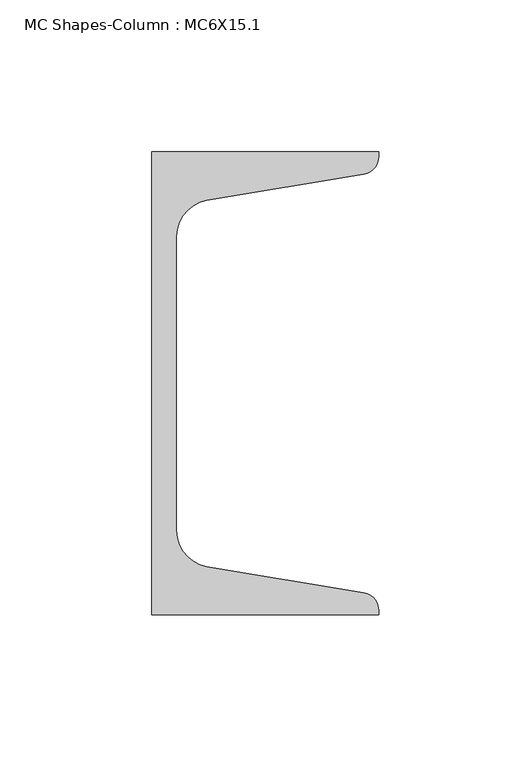
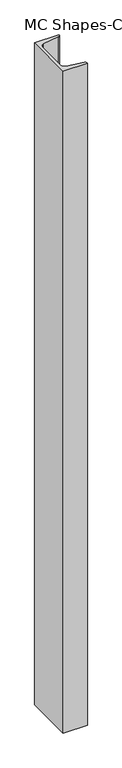
"""IFC4 building model written with IfcOpenShell, lengths in millimetres: column geometry, MC Shapes-Column : MC6X15.1."""

from ifc_helpers import new_model, si_unit, point, frame, frame_2d, origin, place, context, project, spatial, polyline, circle_curve, trimmed, segment, composite_curve, outline, extrude, source, transform, mapped, element, save


def mc_shapes_column_mc6x15_1_878b4d87(model_context):
    return source(origin(), model_context, "Body", "SweptSolid", [
        extrude(outline(composite_curve([segment(polyline([(-23.876, -76.2), (-23.876, 76.2), (50.8, 76.2), (50.8, 74.7994369)]), True, "CONTINUOUS"), segment(trimmed(circle_curve(frame_2d((44.7675, 74.7994369)), 6.0325), [point((50.8, 74.7994369))], [point((45.7592388, 68.8490159))], False, "CARTESIAN"), True, "CONTINUOUS"), segment(polyline([(45.7592388, 68.8490159), (-5.7680776, 60.2611126)]), True, "CONTINUOUS"), segment(trimmed(circle_curve(frame_2d((-3.7846, 48.3602706)), 12.065), [point((-5.7680776, 60.2611126))], [point((-15.8496, 48.3602706))], True, "CARTESIAN"), True, "CONTINUOUS"), segment(polyline([(-15.8496, 48.3602706), (-15.8496, -48.3602706)]), True, "CONTINUOUS"), segment(trimmed(circle_curve(frame_2d((-3.7846, -48.3602706)), 12.065), [point((-15.8496, -48.3602706))], [point((-5.7680776, -60.2611126))], True, "CARTESIAN"), True, "CONTINUOUS"), segment(polyline([(-5.7680776, -60.2611126), (45.7592388, -68.8490159)]), True, "CONTINUOUS"), segment(trimmed(circle_curve(frame_2d((44.7675, -74.7994369)), 6.0325), [point((45.7592388, -68.8490159))], [point((50.8, -74.7994369))], False, "CARTESIAN"), True, "CONTINUOUS"), segment(polyline([(50.8, -74.7994369), (50.8, -76.2), (-23.876, -76.2)]), True, "CONTINUOUS")], self_intersect=False)), frame((0.0, 0.0, 4721.225), z_axis=(0.0, 0.0, 1.0), x_axis=(1.0, 0.0, 0.0)), (0.0, 0.0, 1.0), 2162.175),
    ])


if __name__ == "__main__":
    model = new_model("IFC4")
    model_context = context("Model", 3, world=origin())
    ifc_project = project(units=[si_unit("LENGTHUNIT", "METRE", prefix="MILLI")], contexts=[model_context])
    site = spatial("IfcSite", under=ifc_project)
    building = spatial("IfcBuilding", under=site)
    placement = place(None, origin())
    mc_shapes_column_mc6x15_1_shape = mc_shapes_column_mc6x15_1_878b4d87(model_context)
    element("IfcColumn", 1, ObjectType="MC Shapes-Column : MC6X15.1", at=placement, inside=building, context=model_context, shape_type="MappedRepresentation", body=[
        mapped(mc_shapes_column_mc6x15_1_shape, transform((0.0, 0.0, 0.0), x_axis=(1.0, 0.0, 0.0), y_axis=(0.0, 1.0, 0.0), z_axis=(0.0, 0.0, 1.0))),
    ])
    save(model, "model.ifc")

# Revit data of these elements
# Type "MC Shapes-Column : MC6X15.1"
#   Section Name Key = "MC6X15.1"
#   Assembly Code = "B10"
#   Width = 2.940"
#   Web Thickness = 0.316"
#   Web Fillet = 0.475"
#   Warping Constant = 20.50 in⁶
#   Torsional Moment of Inertia = 0.285 in⁴
#   Sloped Flange Angle = 9.46234°
#   Section Area = 4.44 in²
#   Plastic Modulus weak axis = 3.30 in³
#   Plastic Modulus strong axis = 9.83 in³
#   Nominal Weight = 15.10 lbf/ft
#   Moment of Inertia weak axis = 3.46 in⁴
#   Moment of Inertia strong axis = 24.90 in⁴
#   Height = 6.000"
#   Flange Thickness Location = 1.312"
#   Flange Thickness = 0.475"
#   Flange Fillet = 0.2375"
#   Elastic Modulus weak axis = 1.73 in³
#   Elastic Modulus strong axis = 8.30 in³
#   Centroid Vertical = 3.000"
#   Centroid Horizontal = 0.940"
#   Bolt Spacing = 0' - 1 3/4"
#   Structural Material [instance default] = Steel ASTM A36
#   Principal Axes Angle = 0
# Element 1 (IfcColumn, "MC Shapes-Column : MC6X15.1")
#   Structural Material = Metal - Steel - ASTM A992
#   Materials on its faces: "Metal - Steel - ASTM A992"
# Materials
#   "Steel ASTM A36": class "Metal", colour RGB 199 199 199, transparency 0, Description = "Structural steel, ASTM A36 Grade B, mill finish", Cost = 0
#   "Metal - Steel - ASTM A992": class "Metal", colour RGB 255 128 0, transparency 0
